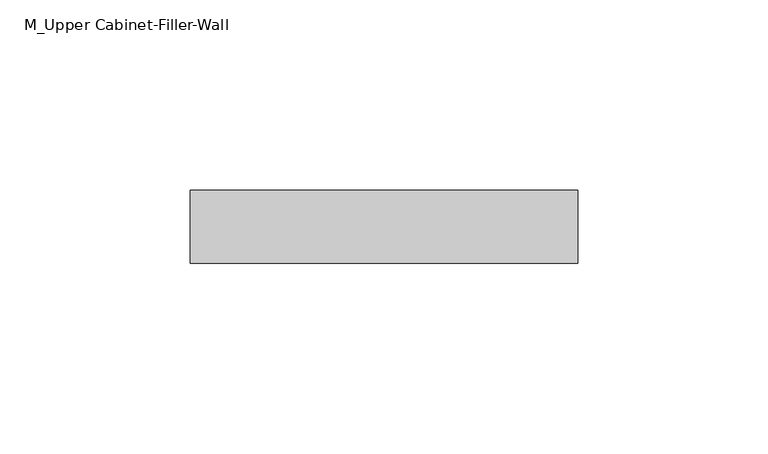
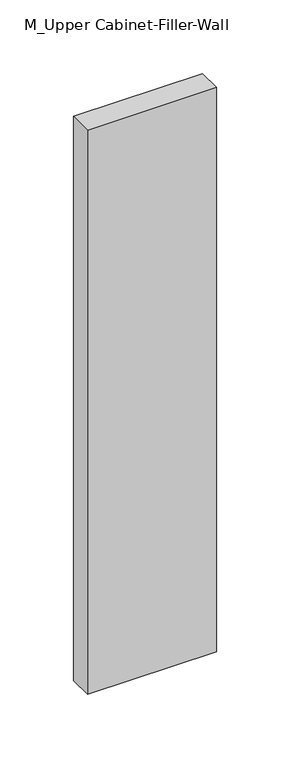
"""IFC4 building model written with IfcOpenShell, lengths in millimetres: furniture geometry, M_Upper Cabinet-Filler-Wall : Fverticle1."""

from ifc_helpers import new_model, si_unit, frame, origin, place, context, project, spatial, polyline, outline, extrude, source, transform, mapped, element, save


def m_upper_cabinet_filler_wall_c56b41ac(model_context):
    return source(origin(), model_context, "Body", "SweptSolid", [
        extrude(outline(polyline([(-21.0288372, 38.1), (-21.0288372, 57.15), (80.5711628, 57.15), (80.5711628, 38.1), (-21.0288372, 38.1)])), frame((0.0, 0.0, 1531.6875), z_axis=(0.0, 0.0, 1.0), x_axis=(1.0, 0.0, 0.0)), (0.0, 0.0, 1.0), 468.3125),
    ])


if __name__ == "__main__":
    model = new_model("IFC4")
    model_context = context("Model", 3, world=origin())
    ifc_project = project(units=[si_unit("LENGTHUNIT", "METRE", prefix="MILLI")], contexts=[model_context])
    site = spatial("IfcSite", under=ifc_project)
    building = spatial("IfcBuilding", under=site)
    placement = place(None, origin())
    m_upper_cabinet_filler_wall_shape = m_upper_cabinet_filler_wall_c56b41ac(model_context)
    element("IfcFurniture", 1, ObjectType="M_Upper Cabinet-Filler-Wall : Fverticle1", at=placement, inside=building, context=model_context, shape_type="MappedRepresentation", body=[
        mapped(m_upper_cabinet_filler_wall_shape, transform((0.0, 0.0, 0.0), x_axis=(1.0, 0.0, 0.0), y_axis=(0.0, 1.0, 0.0), z_axis=(0.0, 0.0, 1.0))),
    ])
    save(model, "model.ifc")

# Revit data of these elements
# Type "M_Upper Cabinet-Filler-Wall : Fverticle1"
#   Depth = 0' - 1"
#   Height = 1' - 6 7/16"
#   Top Of Cabinet = 6' - 6.74016"
#   Width = 0' - 4"
#   Cabinet Material = none
#   Default Elevation = 0
# Element 1 (IfcFurniture, "M_Upper Cabinet-Filler-Wall : Fverticle1")
#   Materials on its faces: "Cabinets"
# Materials
#   "Cabinets": class "Miscellaneous", colour RGB 249 249 249, transparency 0
